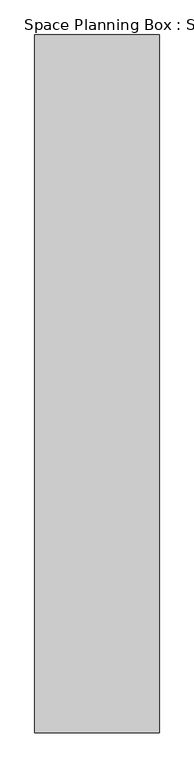
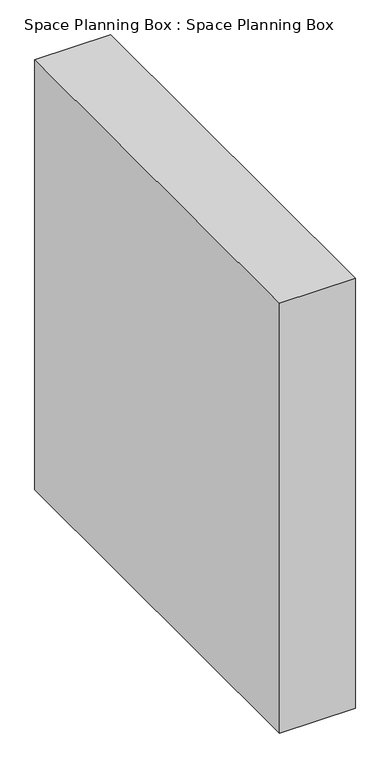
"""IFC4 building model written with IfcOpenShell, lengths in millimetres: proxy geometry, Space Planning Box : Space Planning Box."""

from ifc_helpers import new_model, si_unit, origin, origin_with_axes, place, context, project, spatial, polyline, outline, extrude, source, transform, mapped, element, save


def space_planning_box_space_planning_box_a556ef48(model_context):
    return source(origin(), model_context, "Body", "SweptSolid", [
        extrude(outline(polyline([(500.0, 2800.0), (500.0, -2800.0), (-500.0, -2800.0), (-500.0, 2800.0), (500.0, 2800.0)])), origin_with_axes(), (0.0, 0.0, 1.0), 6000.0),
    ])


if __name__ == "__main__":
    model = new_model("IFC4")
    model_context = context("Model", 3, world=origin())
    ifc_project = project(units=[si_unit("LENGTHUNIT", "METRE", prefix="MILLI")], contexts=[model_context])
    site = spatial("IfcSite", under=ifc_project)
    building = spatial("IfcBuilding", under=site)
    placement = place(None, origin())
    space_planning_box_space_planning_box_shape = space_planning_box_space_planning_box_a556ef48(model_context)
    element("IfcBuildingElementProxy", 1, Name="Space Planning Box : Space Planning Box", ObjectType="Space Planning Box : Space Planning Box", at=placement, inside=building, context=model_context, shape_type="MappedRepresentation", body=[
        mapped(space_planning_box_space_planning_box_shape, transform((0.0, 0.0, 0.0), x_axis=(1.0, 0.0, 0.0), y_axis=(0.0, 1.0, 0.0), z_axis=(0.0, 0.0, 1.0))),
    ])
    save(model, "model.ifc")

# Revit data of these elements
# Type "Space Planning Box : Space Planning Box"
#   Type Comments = "..."
#   Room Name [instance default] = "?"
#   Assembly Code = "..."
#   Width [instance default] = 1524 mm
#   Program Area [instance default] = 0 m²
#   Length [instance default] = 1524 mm
#   Height [instance default] = 1524 mm
#   Area [instance default] = 2.32258 m²
#   Fill Color [instance default] = Cyan
#   Default Elevation = 0
# Element 1 (IfcBuildingElementProxy, "Space Planning Box : Space Planning Box")
#   Room Name = "Shower Room (M)"
#   Width = 1000 mm
#   Program Area = 31.5 m²
#   Length = 5600 mm
#   Height = 6000 mm
#   Area = 5.6 m²
#   Fill Color = Lavender
#   Materials on its faces: "Lavender"
# Materials
#   "Cyan": class "Generic", colour RGB 0 255 255, transparency 0.2, Cost = 0
#   "Lavender": class "Generic", colour RGB 186 85 211, transparency 0.2, Cost = 0
